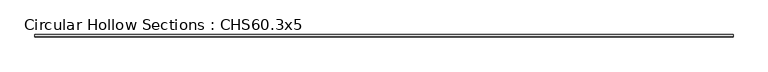
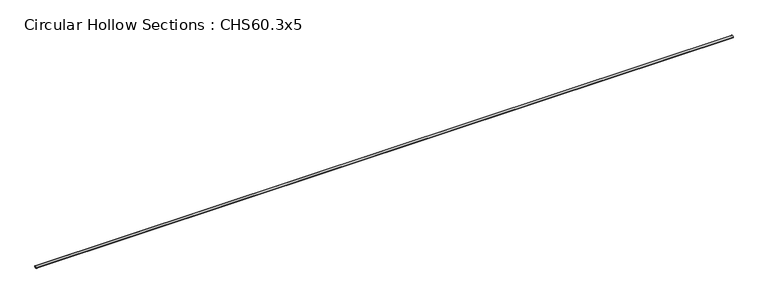
"""IFC4 building model written with IfcOpenShell, lengths in millimetres: beam geometry, Circular Hollow Sections : CHS60.3x5."""

import ifcopenshell
import ifcopenshell.guid

model = None  # the IFC model being written
_history = None  # IfcOwnerHistory: only IFC2X3 demands one
_inside = {}  # id of a spatial element -> (the spatial element, [elements in it])
_under = {}  # id of a project, library or spatial element -> (it, [spatial elements below it])
_declared = {}  # id of a project -> (the project, [libraries it declares])
_typed = {}  # id of a type object -> (the type object, [elements of that type])
_made_of = {}  # id of a material, layer set ... -> (it, [elements and type objects made of it])


def new_model(schema):
    """Start an empty IFC model of exactly this schema.

    Asked for "IFC4X3", IfcOpenShell would pick the latest addendum, in which some entities
    have other attributes; the version numbers below select the first issue.
    IFC2X3 requires an IfcOwnerHistory on every rooted entity: one is made here for all.
    """
    global model, _history
    if schema == "IFC4X3":
        model = ifcopenshell.file(schema_version=(4, 3, 0, 0))
    else:
        model = ifcopenshell.file(schema=schema)
    _inside.clear()
    _under.clear()
    _declared.clear()
    _typed.clear()
    _made_of.clear()
    _history = None
    if model.schema == "IFC2X3":
        org = make("IfcOrganization", Name="unknown")
        user = make(
            "IfcPersonAndOrganization",
            ThePerson=make("IfcPerson", FamilyName="unknown"),
            TheOrganization=org,
        )
        app = make(
            "IfcApplication",
            ApplicationDeveloper=org,
            Version="unknown",
            ApplicationFullName="unknown",
            ApplicationIdentifier="unknown",
        )
        _history = make(
            "IfcOwnerHistory",
            OwningUser=user,
            OwningApplication=app,
            ChangeAction="ADDED",
            CreationDate=0,
        )
    return model


def make(cls, **values):
    """One entity of the class cls with the attributes given. An attribute that is None is left unset."""
    return model.create_entity(
        cls, **{name: value for name, value in values.items() if value is not None}
    )


def rooted(cls, **values):
    """An entity with a GlobalId (a new one), such as an element, a storey or a relation."""
    return make(cls, GlobalId=ifcopenshell.guid.new(), OwnerHistory=_history, **values)


def si_unit(unit_type, name, prefix=None):
    """IfcSIUnit, for example si_unit("LENGTHUNIT", "METRE", prefix="MILLI")."""
    return make("IfcSIUnit", UnitType=unit_type, Prefix=prefix, Name=name)


def assignment(units):
    """IfcUnitAssignment: the units of a project."""
    return None if units is None else make("IfcUnitAssignment", Units=units)


def point(xyz):
    """IfcCartesianPoint."""
    return None if xyz is None else make("IfcCartesianPoint", Coordinates=xyz)


def direction(xyz):
    """IfcDirection."""
    return None if xyz is None else make("IfcDirection", DirectionRatios=xyz)


def frame(location, z_axis=None, x_axis=None):
    """IfcAxis2Placement3D, a coordinate frame: its origin and axes. An axis left out is left unset."""
    return make(
        "IfcAxis2Placement3D",
        Location=point(location),
        Axis=direction(z_axis),
        RefDirection=direction(x_axis),
    )


def frame_2d(location, x_axis=None):
    """IfcAxis2Placement2D, a coordinate frame in the plane: its origin and x axis."""
    return make(
        "IfcAxis2Placement2D", Location=point(location), RefDirection=direction(x_axis)
    )


def origin():
    """The frame at (0, 0, 0) with its axes left unset."""
    return frame((0.0, 0.0, 0.0))


def origin_2d():
    """The frame at (0, 0) in the plane with its x axis left unset."""
    return frame_2d((0.0, 0.0))


def place(relative_to, where):
    """IfcLocalPlacement: puts the frame where relative to a parent placement (None: the world)."""
    return make(
        "IfcLocalPlacement", PlacementRelTo=relative_to, RelativePlacement=where
    )


def context(
    kind, dimensions, precision=None, world=None, true_north=None, identifier=None
):
    """IfcGeometricRepresentationContext, for example the 3D "Model" context."""
    return make(
        "IfcGeometricRepresentationContext",
        ContextIdentifier=identifier,
        ContextType=kind,
        CoordinateSpaceDimension=dimensions,
        Precision=precision,
        WorldCoordinateSystem=world,
        TrueNorth=true_north,
    )


def project(units=None, contexts=None):
    """IfcProject with its units and contexts."""
    return rooted(
        "IfcProject",
        Name="project",
        RepresentationContexts=contexts,
        UnitsInContext=assignment(units),
    )


def spatial(cls, under=None, at=None, **own):
    """A site, building, storey or space (cls), placed at a placement, below another one or the project."""
    s = rooted(cls, ObjectPlacement=at, **own)
    if under is not None:
        _under.setdefault(under.id(), (under, []))[1].append(s)
    return s


def circle_curve(where, radius):
    """IfcCircle in the frame where."""
    return make("IfcCircle", Position=where, Radius=radius)


def trimmed(basis, trim1, trim2, sense, master):
    """IfcTrimmedCurve: the piece of a basis curve between two trims."""
    return make(
        "IfcTrimmedCurve",
        BasisCurve=basis,
        Trim1=trim1,
        Trim2=trim2,
        SenseAgreement=sense,
        MasterRepresentation=master,
    )


def segment(curve, same_sense, transition):
    """IfcCompositeCurveSegment."""
    return make(
        "IfcCompositeCurveSegment",
        Transition=transition,
        SameSense=same_sense,
        ParentCurve=curve,
    )


def composite_curve(segments, self_intersect=None):
    """IfcCompositeCurve: segments joined end to end."""
    return make("IfcCompositeCurve", Segments=segments, SelfIntersect=self_intersect)


def outline(outer, holes=None, kind="AREA"):
    """IfcArbitraryClosedProfileDef: a profile drawn as a closed curve; with holes, ...WithVoids."""
    if holes is None:
        return make("IfcArbitraryClosedProfileDef", ProfileType=kind, OuterCurve=outer)
    return make(
        "IfcArbitraryProfileDefWithVoids",
        ProfileType=kind,
        OuterCurve=outer,
        InnerCurves=holes,
    )


def extrude(swept, where, along, depth):
    """IfcExtrudedAreaSolid: the profile swept, set in the frame where, extruded along a direction by depth."""
    return make(
        "IfcExtrudedAreaSolid",
        SweptArea=swept,
        Position=where,
        ExtrudedDirection=direction(along),
        Depth=depth,
    )


def shape(context_of_items, identifier, shape_type, items):
    """IfcShapeRepresentation: the items that make up one representation, for example the "Body"."""
    return make(
        "IfcShapeRepresentation",
        ContextOfItems=context_of_items,
        RepresentationIdentifier=identifier,
        RepresentationType=shape_type,
        Items=items,
    )


def source(mapping_origin, context_of_items, identifier, shape_type, items):
    """IfcRepresentationMap: a shape defined once, which mapped items show again and again."""
    return make(
        "IfcRepresentationMap",
        MappingOrigin=mapping_origin,
        MappedRepresentation=shape(context_of_items, identifier, shape_type, items),
    )


def transform(
    local_origin,
    x_axis=None,
    y_axis=None,
    z_axis=None,
    scale=None,
    scale2=None,
    scale3=None,
    uniform=True,
):
    """IfcCartesianTransformationOperator3D, or its non-uniform kind. x_axis, y_axis, z_axis: its Axis1, 2, 3."""
    if uniform:
        return make(
            "IfcCartesianTransformationOperator3D",
            Axis1=direction(x_axis),
            Axis2=direction(y_axis),
            LocalOrigin=point(local_origin),
            Scale=scale,
            Axis3=direction(z_axis),
        )
    return make(
        "IfcCartesianTransformationOperator3DnonUniform",
        Axis1=direction(x_axis),
        Axis2=direction(y_axis),
        LocalOrigin=point(local_origin),
        Scale=scale,
        Axis3=direction(z_axis),
        Scale2=scale2,
        Scale3=scale3,
    )


def mapped(mapping_source, mapping_target):
    """IfcMappedItem: shows the shape of a source again, moved by a transform."""
    return make(
        "IfcMappedItem", MappingSource=mapping_source, MappingTarget=mapping_target
    )


def made_of(thing, what):
    """Note that an element or type object is made of a material, layer set ...; save() writes the relation."""
    if what is not None:
        _made_of.setdefault(what.id(), (what, []))[1].append(thing)
    return thing


def element(
    cls,
    number,
    at=None,
    inside=None,
    cuts=None,
    type_object=None,
    material=None,
    context=None,
    identifier="Body",
    shape_type=None,
    held_by="IfcProductDefinitionShape",
    body=None,
    shapes=None,
    **own,
):
    """One element of the class cls, such as IfcWall. Its Tag is "e" and its number.

    at: its placement. inside: the storey or other place that contains it. cuts: it is an
    opening in that element (IfcRelVoidsElement). A single representation is given by context,
    identifier, shape_type and body (its items); several are given by shapes. held_by: the class
    of the entity that holds the representations. save() writes the other relations.
    """
    e = rooted(cls, Tag="e%d" % number, ObjectPlacement=at, **own)
    if body is not None:
        shapes = [shape(context, identifier, shape_type, body)]
    if shapes is not None:
        e.Representation = make(held_by, Representations=shapes)
    if inside is not None:
        _inside.setdefault(inside.id(), (inside, []))[1].append(e)
    if cuts is not None:
        rooted(
            "IfcRelVoidsElement", RelatingBuildingElement=cuts, RelatedOpeningElement=e
        )
    if type_object is not None:
        _typed.setdefault(type_object.id(), (type_object, []))[1].append(e)
    return made_of(e, material)


def aggregate(whole, parts):
    """IfcRelAggregates: a whole, such as a stair, and the parts it consists of."""
    return rooted("IfcRelAggregates", RelatingObject=whole, RelatedObjects=parts)


def save(model, path):
    """Write the relations noted so far, then the file.

    IfcRelAggregates (storeys below a building ...), IfcRelContainedInSpatialStructure (elements
    in a storey), IfcRelDefinesByType, IfcRelAssociatesMaterial and IfcRelDeclares: one each for
    every whole, place, type object, material and project.
    """
    for whole, parts in _under.values():
        aggregate(whole, parts)
    for where, things in _inside.values():
        rooted(
            "IfcRelContainedInSpatialStructure",
            RelatedElements=things,
            RelatingStructure=where,
        )
    for kind, things in _typed.values():
        rooted("IfcRelDefinesByType", RelatedObjects=things, RelatingType=kind)
    for what, things in _made_of.values():
        rooted("IfcRelAssociatesMaterial", RelatedObjects=things, RelatingMaterial=what)
    for by, libraries in _declared.values():
        rooted("IfcRelDeclares", RelatingContext=by, RelatedDefinitions=libraries)
    model.write(path)


def circular_hollow_sections_chs60_3x5_ee2473de(model_context):
    return source(origin(), model_context, "Body", "SweptSolid", [
        extrude(outline(composite_curve([segment(trimmed(circle_curve(origin_2d(), 30.15), [point((-30.15, 0.0))], [point((30.15, 0.0))], False, "CARTESIAN"), True, "CONTINUOUS"), segment(trimmed(circle_curve(origin_2d(), 30.15), [point((30.15, 0.0))], [point((-30.15, 0.0))], False, "CARTESIAN"), True, "CONTINUOUS")], self_intersect=False), holes=[composite_curve([segment(trimmed(circle_curve(origin_2d(), 25.15), [point((25.15, 0.0))], [point((-25.15, 0.0))], True, "CARTESIAN"), True, "CONTINUOUS"), segment(trimmed(circle_curve(origin_2d(), 25.15), [point((-25.15, 0.0))], [point((25.15, 0.0))], True, "CARTESIAN"), True, "CONTINUOUS")], self_intersect=False)]), frame((-9000.0, 0.0, 0.0), z_axis=(1.0, 0.0, 0.0), x_axis=(0.0, 1.0, 0.0)), (0.0, 0.0, 1.0), 18000.0),
    ])


if __name__ == "__main__":
    model = new_model("IFC4")
    model_context = context("Model", 3, world=origin())
    ifc_project = project(units=[si_unit("LENGTHUNIT", "METRE", prefix="MILLI")], contexts=[model_context])
    site = spatial("IfcSite", under=ifc_project)
    building = spatial("IfcBuilding", under=site)
    placement = place(None, origin())
    circular_hollow_sections_chs60_3x5_shape = circular_hollow_sections_chs60_3x5_ee2473de(model_context)
    element("IfcBeam", 1, ObjectType="Circular Hollow Sections : CHS60.3x5", at=placement, inside=building, context=model_context, shape_type="MappedRepresentation", body=[
        mapped(circular_hollow_sections_chs60_3x5_shape, transform((0.0, 0.0, 0.0), x_axis=(1.0, 0.0, 0.0), y_axis=(0.0, 1.0, 0.0), z_axis=(0.0, 0.0, 1.0))),
    ])
    save(model, "model.ifc")

# Revit data of these elements
# Type "Circular Hollow Sections : CHS60.3x5"
#   Description = "Hollow Core Steel Roof Truss Member"
#   Type Comments = "Steel 50-355"
#   Assembly Code = "F10"
#   t = 5 mm
#   W = 0.00682
#   Start Extension Calculation [instance default] = 3000 mm
#   Start Extension [instance default] = -12.7 mm
#   Length [instance default] = 1500 mm
#   OD = 60.3 mm
#   End Extension Calculation [instance default] = 3000 mm
#   End Extension [instance default] = -12.7 mm
#   A = 0.000869 m²
#   Structural Material [instance default] = Metal - Steel 50-355
# Element 1 (IfcBeam, "Circular Hollow Sections : CHS60.3x5")
#   Materials on its faces: "Metal - Steel 50-355"
# Materials
#   "Metal - Steel 50-355": class "Metal", colour RGB 247 247 247, transparency 0
